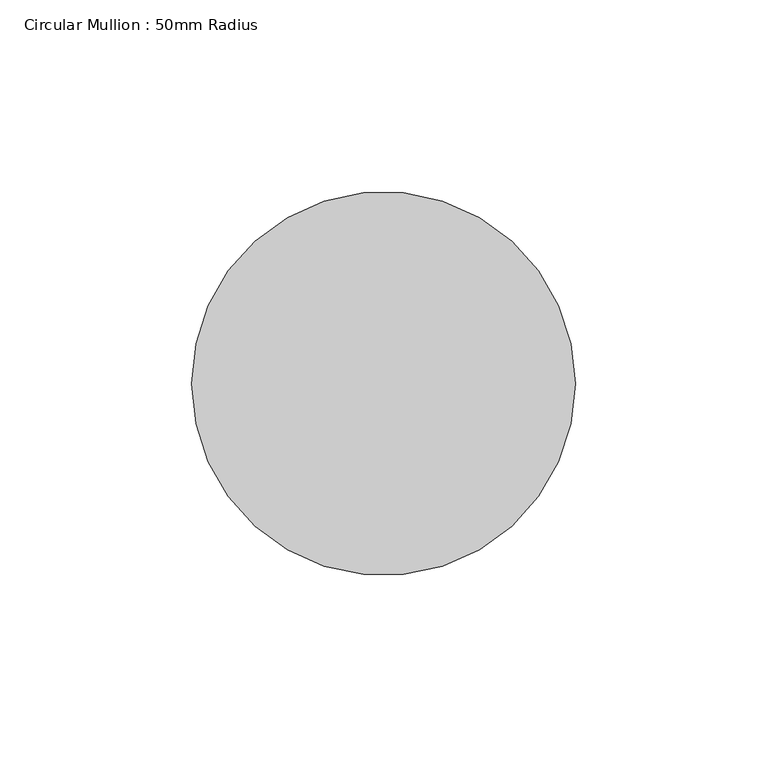
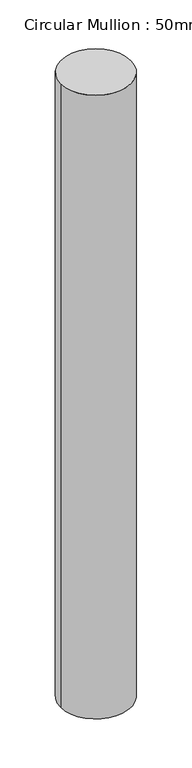
"""IFC4 building model written with IfcOpenShell, lengths in millimetres: member geometry, Circular Mullion : 50mm Radius."""

from ifc_helpers import new_model, si_unit, point, frame, origin, origin_2d, place, context, project, spatial, circle_curve, trimmed, segment, composite_curve, outline, extrude, source, transform, mapped, element, save


def circular_mullion_50mm_radius_848d774e(model_context):
    return source(origin(), model_context, "Body", "SweptSolid", [
        extrude(outline(composite_curve([segment(trimmed(circle_curve(origin_2d(), 50.0), [point((50.0, 0.0))], [point((-50.0, 0.0))], False, "CARTESIAN"), True, "CONTINUOUS"), segment(trimmed(circle_curve(origin_2d(), 50.0), [point((-50.0, 0.0))], [point((50.0, 0.0))], False, "CARTESIAN"), True, "CONTINUOUS")], self_intersect=False)), frame((0.0, 0.0, -940.2774687), z_axis=(0.0, 0.0, 1.0), x_axis=(1.0, 0.0, 0.0)), (0.0, 0.0, 1.0), 940.2774687),
    ])


if __name__ == "__main__":
    model = new_model("IFC4")
    model_context = context("Model", 3, world=origin())
    ifc_project = project(units=[si_unit("LENGTHUNIT", "METRE", prefix="MILLI")], contexts=[model_context])
    site = spatial("IfcSite", under=ifc_project)
    building = spatial("IfcBuilding", under=site)
    placement = place(None, origin())
    circular_mullion_50mm_radius_shape = circular_mullion_50mm_radius_848d774e(model_context)
    element("IfcMember", 1, ObjectType="Circular Mullion : 50mm Radius", at=placement, inside=building, context=model_context, shape_type="MappedRepresentation", body=[
        mapped(circular_mullion_50mm_radius_shape, transform((0.0, 0.0, 0.0), x_axis=(1.0, 0.0, 0.0), y_axis=(0.0, 1.0, 0.0), z_axis=(0.0, 0.0, 1.0))),
    ])
    save(model, "model.ifc")

# Revit data of these elements
# Type "Circular Mullion : 50mm Radius"
#   built-in parameter 1007350 = 0.164042 (stored number, unit not read)
# Element 1 (IfcMember, "Circular Mullion : 50mm Radius")
#   Materials on its faces: "Aluminium"
# Materials
#   "Aluminium": class "Metal", colour RGB 247 247 247, transparency 0, Description = "Aluminium 6061", Cost = 0
